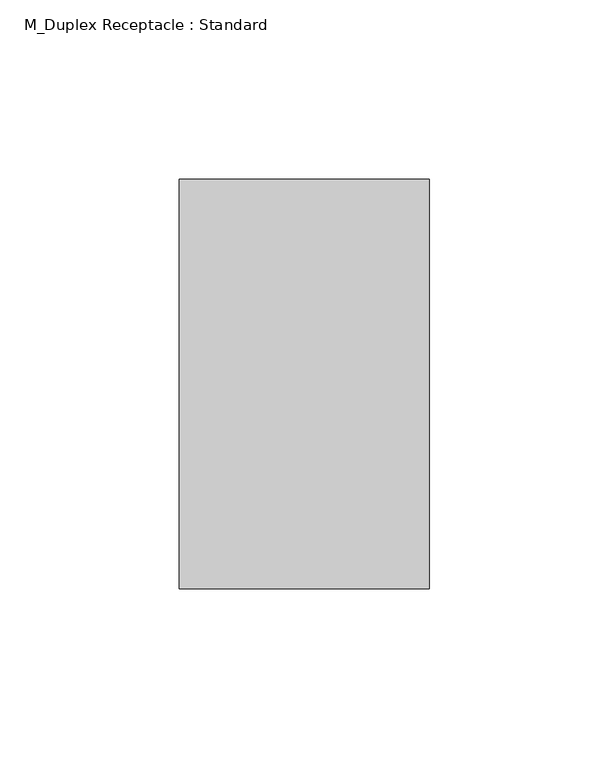
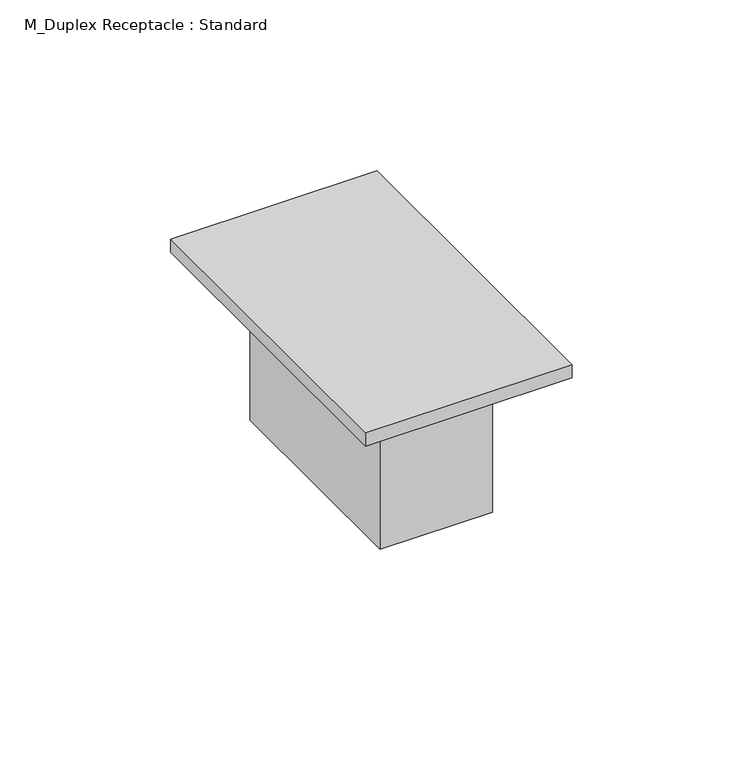
"""IFC4 building model written with IfcOpenShell, lengths in millimetres: proxy geometry, M_Duplex Receptacle : Standard."""

import ifcopenshell
import ifcopenshell.guid

model = None  # the IFC model being written
_history = None  # IfcOwnerHistory: only IFC2X3 demands one
_inside = {}  # id of a spatial element -> (the spatial element, [elements in it])
_under = {}  # id of a project, library or spatial element -> (it, [spatial elements below it])
_declared = {}  # id of a project -> (the project, [libraries it declares])
_typed = {}  # id of a type object -> (the type object, [elements of that type])
_made_of = {}  # id of a material, layer set ... -> (it, [elements and type objects made of it])


def new_model(schema):
    """Start an empty IFC model of exactly this schema.

    Asked for "IFC4X3", IfcOpenShell would pick the latest addendum, in which some entities
    have other attributes; the version numbers below select the first issue.
    IFC2X3 requires an IfcOwnerHistory on every rooted entity: one is made here for all.
    """
    global model, _history
    if schema == "IFC4X3":
        model = ifcopenshell.file(schema_version=(4, 3, 0, 0))
    else:
        model = ifcopenshell.file(schema=schema)
    _inside.clear()
    _under.clear()
    _declared.clear()
    _typed.clear()
    _made_of.clear()
    _history = None
    if model.schema == "IFC2X3":
        org = make("IfcOrganization", Name="unknown")
        user = make(
            "IfcPersonAndOrganization",
            ThePerson=make("IfcPerson", FamilyName="unknown"),
            TheOrganization=org,
        )
        app = make(
            "IfcApplication",
            ApplicationDeveloper=org,
            Version="unknown",
            ApplicationFullName="unknown",
            ApplicationIdentifier="unknown",
        )
        _history = make(
            "IfcOwnerHistory",
            OwningUser=user,
            OwningApplication=app,
            ChangeAction="ADDED",
            CreationDate=0,
        )
    return model


def make(cls, **values):
    """One entity of the class cls with the attributes given. An attribute that is None is left unset."""
    return model.create_entity(
        cls, **{name: value for name, value in values.items() if value is not None}
    )


def rooted(cls, **values):
    """An entity with a GlobalId (a new one), such as an element, a storey or a relation."""
    return make(cls, GlobalId=ifcopenshell.guid.new(), OwnerHistory=_history, **values)


def si_unit(unit_type, name, prefix=None):
    """IfcSIUnit, for example si_unit("LENGTHUNIT", "METRE", prefix="MILLI")."""
    return make("IfcSIUnit", UnitType=unit_type, Prefix=prefix, Name=name)


def assignment(units):
    """IfcUnitAssignment: the units of a project."""
    return None if units is None else make("IfcUnitAssignment", Units=units)


def point(xyz):
    """IfcCartesianPoint."""
    return None if xyz is None else make("IfcCartesianPoint", Coordinates=xyz)


def direction(xyz):
    """IfcDirection."""
    return None if xyz is None else make("IfcDirection", DirectionRatios=xyz)


def frame(location, z_axis=None, x_axis=None):
    """IfcAxis2Placement3D, a coordinate frame: its origin and axes. An axis left out is left unset."""
    return make(
        "IfcAxis2Placement3D",
        Location=point(location),
        Axis=direction(z_axis),
        RefDirection=direction(x_axis),
    )


def origin():
    """The frame at (0, 0, 0) with its axes left unset."""
    return frame((0.0, 0.0, 0.0))


def origin_with_axes():
    """The frame at (0, 0, 0) with the z axis (0, 0, 1) and the x axis (1, 0, 0) written out."""
    return frame((0.0, 0.0, 0.0), z_axis=(0.0, 0.0, 1.0), x_axis=(1.0, 0.0, 0.0))


def place(relative_to, where):
    """IfcLocalPlacement: puts the frame where relative to a parent placement (None: the world)."""
    return make(
        "IfcLocalPlacement", PlacementRelTo=relative_to, RelativePlacement=where
    )


def context(
    kind, dimensions, precision=None, world=None, true_north=None, identifier=None
):
    """IfcGeometricRepresentationContext, for example the 3D "Model" context."""
    return make(
        "IfcGeometricRepresentationContext",
        ContextIdentifier=identifier,
        ContextType=kind,
        CoordinateSpaceDimension=dimensions,
        Precision=precision,
        WorldCoordinateSystem=world,
        TrueNorth=true_north,
    )


def project(units=None, contexts=None):
    """IfcProject with its units and contexts."""
    return rooted(
        "IfcProject",
        Name="project",
        RepresentationContexts=contexts,
        UnitsInContext=assignment(units),
    )


def spatial(cls, under=None, at=None, **own):
    """A site, building, storey or space (cls), placed at a placement, below another one or the project."""
    s = rooted(cls, ObjectPlacement=at, **own)
    if under is not None:
        _under.setdefault(under.id(), (under, []))[1].append(s)
    return s


def polyline(points):
    """IfcPolyline through the points."""
    return make("IfcPolyline", Points=[point(p) for p in points])


def outline(outer, holes=None, kind="AREA"):
    """IfcArbitraryClosedProfileDef: a profile drawn as a closed curve; with holes, ...WithVoids."""
    if holes is None:
        return make("IfcArbitraryClosedProfileDef", ProfileType=kind, OuterCurve=outer)
    return make(
        "IfcArbitraryProfileDefWithVoids",
        ProfileType=kind,
        OuterCurve=outer,
        InnerCurves=holes,
    )


def extrude(swept, where, along, depth):
    """IfcExtrudedAreaSolid: the profile swept, set in the frame where, extruded along a direction by depth."""
    return make(
        "IfcExtrudedAreaSolid",
        SweptArea=swept,
        Position=where,
        ExtrudedDirection=direction(along),
        Depth=depth,
    )


def shape(context_of_items, identifier, shape_type, items):
    """IfcShapeRepresentation: the items that make up one representation, for example the "Body"."""
    return make(
        "IfcShapeRepresentation",
        ContextOfItems=context_of_items,
        RepresentationIdentifier=identifier,
        RepresentationType=shape_type,
        Items=items,
    )


def source(mapping_origin, context_of_items, identifier, shape_type, items):
    """IfcRepresentationMap: a shape defined once, which mapped items show again and again."""
    return make(
        "IfcRepresentationMap",
        MappingOrigin=mapping_origin,
        MappedRepresentation=shape(context_of_items, identifier, shape_type, items),
    )


def transform(
    local_origin,
    x_axis=None,
    y_axis=None,
    z_axis=None,
    scale=None,
    scale2=None,
    scale3=None,
    uniform=True,
):
    """IfcCartesianTransformationOperator3D, or its non-uniform kind. x_axis, y_axis, z_axis: its Axis1, 2, 3."""
    if uniform:
        return make(
            "IfcCartesianTransformationOperator3D",
            Axis1=direction(x_axis),
            Axis2=direction(y_axis),
            LocalOrigin=point(local_origin),
            Scale=scale,
            Axis3=direction(z_axis),
        )
    return make(
        "IfcCartesianTransformationOperator3DnonUniform",
        Axis1=direction(x_axis),
        Axis2=direction(y_axis),
        LocalOrigin=point(local_origin),
        Scale=scale,
        Axis3=direction(z_axis),
        Scale2=scale2,
        Scale3=scale3,
    )


def mapped(mapping_source, mapping_target):
    """IfcMappedItem: shows the shape of a source again, moved by a transform."""
    return make(
        "IfcMappedItem", MappingSource=mapping_source, MappingTarget=mapping_target
    )


def made_of(thing, what):
    """Note that an element or type object is made of a material, layer set ...; save() writes the relation."""
    if what is not None:
        _made_of.setdefault(what.id(), (what, []))[1].append(thing)
    return thing


def element(
    cls,
    number,
    at=None,
    inside=None,
    cuts=None,
    type_object=None,
    material=None,
    context=None,
    identifier="Body",
    shape_type=None,
    held_by="IfcProductDefinitionShape",
    body=None,
    shapes=None,
    **own,
):
    """One element of the class cls, such as IfcWall. Its Tag is "e" and its number.

    at: its placement. inside: the storey or other place that contains it. cuts: it is an
    opening in that element (IfcRelVoidsElement). A single representation is given by context,
    identifier, shape_type and body (its items); several are given by shapes. held_by: the class
    of the entity that holds the representations. save() writes the other relations.
    """
    e = rooted(cls, Tag="e%d" % number, ObjectPlacement=at, **own)
    if body is not None:
        shapes = [shape(context, identifier, shape_type, body)]
    if shapes is not None:
        e.Representation = make(held_by, Representations=shapes)
    if inside is not None:
        _inside.setdefault(inside.id(), (inside, []))[1].append(e)
    if cuts is not None:
        rooted(
            "IfcRelVoidsElement", RelatingBuildingElement=cuts, RelatedOpeningElement=e
        )
    if type_object is not None:
        _typed.setdefault(type_object.id(), (type_object, []))[1].append(e)
    return made_of(e, material)


def aggregate(whole, parts):
    """IfcRelAggregates: a whole, such as a stair, and the parts it consists of."""
    return rooted("IfcRelAggregates", RelatingObject=whole, RelatedObjects=parts)


def save(model, path):
    """Write the relations noted so far, then the file.

    IfcRelAggregates (storeys below a building ...), IfcRelContainedInSpatialStructure (elements
    in a storey), IfcRelDefinesByType, IfcRelAssociatesMaterial and IfcRelDeclares: one each for
    every whole, place, type object, material and project.
    """
    for whole, parts in _under.values():
        aggregate(whole, parts)
    for where, things in _inside.values():
        rooted(
            "IfcRelContainedInSpatialStructure",
            RelatedElements=things,
            RelatingStructure=where,
        )
    for kind, things in _typed.values():
        rooted("IfcRelDefinesByType", RelatedObjects=things, RelatingType=kind)
    for what, things in _made_of.values():
        rooted("IfcRelAssociatesMaterial", RelatedObjects=things, RelatingMaterial=what)
    for by, libraries in _declared.values():
        rooted("IfcRelDeclares", RelatingContext=by, RelatedDefinitions=libraries)
    model.write(path)


def m_duplex_receptacle_standard_10251bba(model_context):
    return source(origin(), model_context, "Body", "SweptSolid", [
        extrude(outline(polyline([(19.05, 38.1), (19.05, -38.1), (-19.05, -38.1), (-19.05, 38.1), (19.05, 38.1)])), frame((0.0, 0.0, -53.975), z_axis=(0.0, 0.0, 1.0), x_axis=(1.0, 0.0, 0.0)), (0.0, 0.0, 1.0), 53.975),
        extrude(outline(polyline([(34.925, 57.15), (34.925, -57.15), (-34.925, -57.15), (-34.925, 57.15), (34.925, 57.15)])), origin_with_axes(), (0.0, 0.0, 1.0), 4.7625),
    ])


if __name__ == "__main__":
    model = new_model("IFC4")
    model_context = context("Model", 3, world=origin())
    ifc_project = project(units=[si_unit("LENGTHUNIT", "METRE", prefix="MILLI")], contexts=[model_context])
    site = spatial("IfcSite", under=ifc_project)
    building = spatial("IfcBuilding", under=site)
    placement = place(None, origin())
    m_duplex_receptacle_standard_shape = m_duplex_receptacle_standard_10251bba(model_context)
    element("IfcBuildingElementProxy", 1, Name="M_Duplex Receptacle : Standard", ObjectType="M_Duplex Receptacle : Standard", at=placement, inside=building, context=model_context, shape_type="MappedRepresentation", body=[
        mapped(m_duplex_receptacle_standard_shape, transform((0.0, 0.0, 0.0), x_axis=(1.0, 0.0, 0.0), y_axis=(0.0, 1.0, 0.0), z_axis=(0.0, 0.0, 1.0))),
    ])
    save(model, "model.ifc")

# Revit data of these elements
# Type "M_Duplex Receptacle : Standard"
#   Label = ""
#   Switch Voltage = 120 V
#   Load = 180 VA
#   Default Elevation = 460 mm
#   Load Classification = Receptacle
#   Assembly Code = ""
